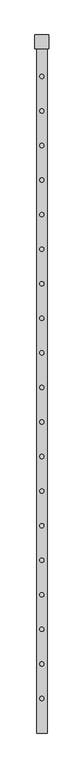
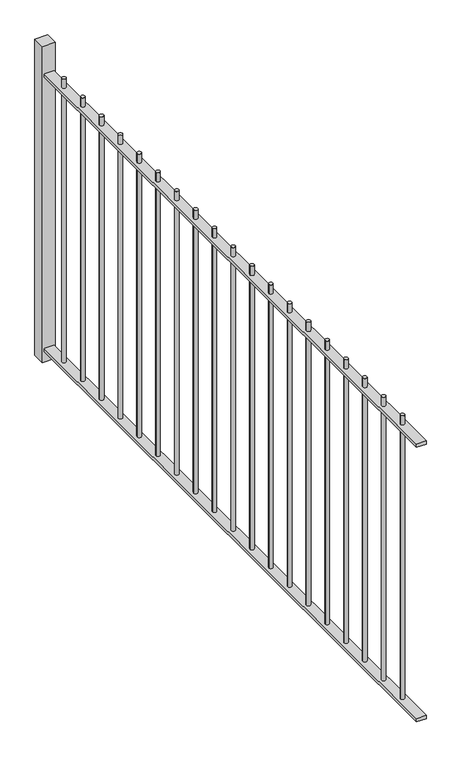
"""IFC4 building model written with IfcOpenShell, lengths in millimetres: railing geometry."""

from ifc_helpers import new_model, si_unit, point, frame, frame_2d, origin, place, context, project, spatial, polyline, circle_curve, trimmed, segment, composite_curve, outline, extrude, source, transform, mapped, element, save


def railing_8eb08526(model_context):
    return source(origin(), model_context, "Body", "SweptSolid", [
        extrude(outline(polyline([(-6549.419961, -16851.1119119), (-6489.419961, -16851.1119119), (-6489.419961, -20851.1119119), (-6549.419961, -20851.1119119), (-6549.419961, -16851.1119119)])), frame((0.0, 0.0, -30.0), z_axis=(0.0, 0.0, 1.0), x_axis=(1.0, 0.0, 0.0)), (0.0, 0.0, 1.0), 20.0),
        extrude(outline(polyline([(-6549.419961, -16851.1119119), (-6489.419961, -16851.1119119), (-6489.419961, -20851.1119119), (-6549.419961, -20851.1119119), (-6549.419961, -16851.1119119)])), frame((0.0, 0.0, 1750.0), z_axis=(0.0, 0.0, 1.0), x_axis=(1.0, 0.0, 0.0)), (0.0, 0.0, 1.0), 20.0),
        extrude(outline(composite_curve([segment(trimmed(circle_curve(frame_2d((-6519.419961, -20651.1119119)), 12.5), [point((-6531.919961, -20651.1119119))], [point((-6506.919961, -20651.1119119))], False, "CARTESIAN"), True, "CONTINUOUS"), segment(trimmed(circle_curve(frame_2d((-6519.419961, -20651.1119119)), 12.5), [point((-6506.919961, -20651.1119119))], [point((-6531.919961, -20651.1119119))], False, "CARTESIAN"), True, "CONTINUOUS")], self_intersect=False)), frame((0.0, 0.0, -10.0), z_axis=(0.0, 0.0, 1.0), x_axis=(1.0, 0.0, 0.0)), (0.0, 0.0, 1.0), 1840.0),
        extrude(outline(composite_curve([segment(trimmed(circle_curve(frame_2d((-6519.419961, -20451.1119119)), 12.5), [point((-6531.919961, -20451.1119119))], [point((-6506.919961, -20451.1119119))], False, "CARTESIAN"), True, "CONTINUOUS"), segment(trimmed(circle_curve(frame_2d((-6519.419961, -20451.1119119)), 12.5), [point((-6506.919961, -20451.1119119))], [point((-6531.919961, -20451.1119119))], False, "CARTESIAN"), True, "CONTINUOUS")], self_intersect=False)), frame((0.0, 0.0, -10.0), z_axis=(0.0, 0.0, 1.0), x_axis=(1.0, 0.0, 0.0)), (0.0, 0.0, 1.0), 1840.0),
        extrude(outline(composite_curve([segment(trimmed(circle_curve(frame_2d((-6519.419961, -20251.1119119)), 12.5), [point((-6531.919961, -20251.1119119))], [point((-6506.919961, -20251.1119119))], False, "CARTESIAN"), True, "CONTINUOUS"), segment(trimmed(circle_curve(frame_2d((-6519.419961, -20251.1119119)), 12.5), [point((-6506.919961, -20251.1119119))], [point((-6531.919961, -20251.1119119))], False, "CARTESIAN"), True, "CONTINUOUS")], self_intersect=False)), frame((0.0, 0.0, -10.0), z_axis=(0.0, 0.0, 1.0), x_axis=(1.0, 0.0, 0.0)), (0.0, 0.0, 1.0), 1840.0),
        extrude(outline(composite_curve([segment(trimmed(circle_curve(frame_2d((-6519.419961, -20051.1119119)), 12.5), [point((-6531.919961, -20051.1119119))], [point((-6506.919961, -20051.1119119))], False, "CARTESIAN"), True, "CONTINUOUS"), segment(trimmed(circle_curve(frame_2d((-6519.419961, -20051.1119119)), 12.5), [point((-6506.919961, -20051.1119119))], [point((-6531.919961, -20051.1119119))], False, "CARTESIAN"), True, "CONTINUOUS")], self_intersect=False)), frame((0.0, 0.0, -10.0), z_axis=(0.0, 0.0, 1.0), x_axis=(1.0, 0.0, 0.0)), (0.0, 0.0, 1.0), 1840.0),
        extrude(outline(composite_curve([segment(trimmed(circle_curve(frame_2d((-6519.419961, -19851.1119119)), 12.5), [point((-6531.919961, -19851.1119119))], [point((-6506.919961, -19851.1119119))], False, "CARTESIAN"), True, "CONTINUOUS"), segment(trimmed(circle_curve(frame_2d((-6519.419961, -19851.1119119)), 12.5), [point((-6506.919961, -19851.1119119))], [point((-6531.919961, -19851.1119119))], False, "CARTESIAN"), True, "CONTINUOUS")], self_intersect=False)), frame((0.0, 0.0, -10.0), z_axis=(0.0, 0.0, 1.0), x_axis=(1.0, 0.0, 0.0)), (0.0, 0.0, 1.0), 1840.0),
        extrude(outline(composite_curve([segment(trimmed(circle_curve(frame_2d((-6519.419961, -19651.1119119)), 12.5), [point((-6531.919961, -19651.1119119))], [point((-6506.919961, -19651.1119119))], False, "CARTESIAN"), True, "CONTINUOUS"), segment(trimmed(circle_curve(frame_2d((-6519.419961, -19651.1119119)), 12.5), [point((-6506.919961, -19651.1119119))], [point((-6531.919961, -19651.1119119))], False, "CARTESIAN"), True, "CONTINUOUS")], self_intersect=False)), frame((0.0, 0.0, -10.0), z_axis=(0.0, 0.0, 1.0), x_axis=(1.0, 0.0, 0.0)), (0.0, 0.0, 1.0), 1840.0),
        extrude(outline(composite_curve([segment(trimmed(circle_curve(frame_2d((-6519.419961, -19451.1119119)), 12.5), [point((-6531.919961, -19451.1119119))], [point((-6506.919961, -19451.1119119))], False, "CARTESIAN"), True, "CONTINUOUS"), segment(trimmed(circle_curve(frame_2d((-6519.419961, -19451.1119119)), 12.5), [point((-6506.919961, -19451.1119119))], [point((-6531.919961, -19451.1119119))], False, "CARTESIAN"), True, "CONTINUOUS")], self_intersect=False)), frame((0.0, 0.0, -10.0), z_axis=(0.0, 0.0, 1.0), x_axis=(1.0, 0.0, 0.0)), (0.0, 0.0, 1.0), 1840.0),
        extrude(outline(composite_curve([segment(trimmed(circle_curve(frame_2d((-6519.419961, -19251.1119119)), 12.5), [point((-6531.919961, -19251.1119119))], [point((-6506.919961, -19251.1119119))], False, "CARTESIAN"), True, "CONTINUOUS"), segment(trimmed(circle_curve(frame_2d((-6519.419961, -19251.1119119)), 12.5), [point((-6506.919961, -19251.1119119))], [point((-6531.919961, -19251.1119119))], False, "CARTESIAN"), True, "CONTINUOUS")], self_intersect=False)), frame((0.0, 0.0, -10.0), z_axis=(0.0, 0.0, 1.0), x_axis=(1.0, 0.0, 0.0)), (0.0, 0.0, 1.0), 1840.0),
        extrude(outline(composite_curve([segment(trimmed(circle_curve(frame_2d((-6519.419961, -19051.1119119)), 12.5), [point((-6531.919961, -19051.1119119))], [point((-6506.919961, -19051.1119119))], False, "CARTESIAN"), True, "CONTINUOUS"), segment(trimmed(circle_curve(frame_2d((-6519.419961, -19051.1119119)), 12.5), [point((-6506.919961, -19051.1119119))], [point((-6531.919961, -19051.1119119))], False, "CARTESIAN"), True, "CONTINUOUS")], self_intersect=False)), frame((0.0, 0.0, -10.0), z_axis=(0.0, 0.0, 1.0), x_axis=(1.0, 0.0, 0.0)), (0.0, 0.0, 1.0), 1840.0),
        extrude(outline(composite_curve([segment(trimmed(circle_curve(frame_2d((-6519.419961, -18851.1119119)), 12.5), [point((-6531.919961, -18851.1119119))], [point((-6506.919961, -18851.1119119))], False, "CARTESIAN"), True, "CONTINUOUS"), segment(trimmed(circle_curve(frame_2d((-6519.419961, -18851.1119119)), 12.5), [point((-6506.919961, -18851.1119119))], [point((-6531.919961, -18851.1119119))], False, "CARTESIAN"), True, "CONTINUOUS")], self_intersect=False)), frame((0.0, 0.0, -10.0), z_axis=(0.0, 0.0, 1.0), x_axis=(1.0, 0.0, 0.0)), (0.0, 0.0, 1.0), 1840.0),
        extrude(outline(composite_curve([segment(trimmed(circle_curve(frame_2d((-6519.419961, -18651.1119119)), 12.5), [point((-6531.919961, -18651.1119119))], [point((-6506.919961, -18651.1119119))], False, "CARTESIAN"), True, "CONTINUOUS"), segment(trimmed(circle_curve(frame_2d((-6519.419961, -18651.1119119)), 12.5), [point((-6506.919961, -18651.1119119))], [point((-6531.919961, -18651.1119119))], False, "CARTESIAN"), True, "CONTINUOUS")], self_intersect=False)), frame((0.0, 0.0, -10.0), z_axis=(0.0, 0.0, 1.0), x_axis=(1.0, 0.0, 0.0)), (0.0, 0.0, 1.0), 1840.0),
        extrude(outline(composite_curve([segment(trimmed(circle_curve(frame_2d((-6519.419961, -18451.1119119)), 12.5), [point((-6531.919961, -18451.1119119))], [point((-6506.919961, -18451.1119119))], False, "CARTESIAN"), True, "CONTINUOUS"), segment(trimmed(circle_curve(frame_2d((-6519.419961, -18451.1119119)), 12.5), [point((-6506.919961, -18451.1119119))], [point((-6531.919961, -18451.1119119))], False, "CARTESIAN"), True, "CONTINUOUS")], self_intersect=False)), frame((0.0, 0.0, -10.0), z_axis=(0.0, 0.0, 1.0), x_axis=(1.0, 0.0, 0.0)), (0.0, 0.0, 1.0), 1840.0),
        extrude(outline(composite_curve([segment(trimmed(circle_curve(frame_2d((-6519.419961, -18251.1119119)), 12.5), [point((-6531.919961, -18251.1119119))], [point((-6506.919961, -18251.1119119))], False, "CARTESIAN"), True, "CONTINUOUS"), segment(trimmed(circle_curve(frame_2d((-6519.419961, -18251.1119119)), 12.5), [point((-6506.919961, -18251.1119119))], [point((-6531.919961, -18251.1119119))], False, "CARTESIAN"), True, "CONTINUOUS")], self_intersect=False)), frame((0.0, 0.0, -10.0), z_axis=(0.0, 0.0, 1.0), x_axis=(1.0, 0.0, 0.0)), (0.0, 0.0, 1.0), 1840.0),
        extrude(outline(composite_curve([segment(trimmed(circle_curve(frame_2d((-6519.419961, -18051.1119119)), 12.5), [point((-6531.919961, -18051.1119119))], [point((-6506.919961, -18051.1119119))], False, "CARTESIAN"), True, "CONTINUOUS"), segment(trimmed(circle_curve(frame_2d((-6519.419961, -18051.1119119)), 12.5), [point((-6506.919961, -18051.1119119))], [point((-6531.919961, -18051.1119119))], False, "CARTESIAN"), True, "CONTINUOUS")], self_intersect=False)), frame((0.0, 0.0, -10.0), z_axis=(0.0, 0.0, 1.0), x_axis=(1.0, 0.0, 0.0)), (0.0, 0.0, 1.0), 1840.0),
        extrude(outline(composite_curve([segment(trimmed(circle_curve(frame_2d((-6519.419961, -17851.1119119)), 12.5), [point((-6531.919961, -17851.1119119))], [point((-6506.919961, -17851.1119119))], False, "CARTESIAN"), True, "CONTINUOUS"), segment(trimmed(circle_curve(frame_2d((-6519.419961, -17851.1119119)), 12.5), [point((-6506.919961, -17851.1119119))], [point((-6531.919961, -17851.1119119))], False, "CARTESIAN"), True, "CONTINUOUS")], self_intersect=False)), frame((0.0, 0.0, -10.0), z_axis=(0.0, 0.0, 1.0), x_axis=(1.0, 0.0, 0.0)), (0.0, 0.0, 1.0), 1840.0),
        extrude(outline(composite_curve([segment(trimmed(circle_curve(frame_2d((-6519.419961, -17651.1119119)), 12.5), [point((-6531.919961, -17651.1119119))], [point((-6506.919961, -17651.1119119))], False, "CARTESIAN"), True, "CONTINUOUS"), segment(trimmed(circle_curve(frame_2d((-6519.419961, -17651.1119119)), 12.5), [point((-6506.919961, -17651.1119119))], [point((-6531.919961, -17651.1119119))], False, "CARTESIAN"), True, "CONTINUOUS")], self_intersect=False)), frame((0.0, 0.0, -10.0), z_axis=(0.0, 0.0, 1.0), x_axis=(1.0, 0.0, 0.0)), (0.0, 0.0, 1.0), 1840.0),
        extrude(outline(composite_curve([segment(trimmed(circle_curve(frame_2d((-6519.419961, -17451.1119119)), 12.5), [point((-6531.919961, -17451.1119119))], [point((-6506.919961, -17451.1119119))], False, "CARTESIAN"), True, "CONTINUOUS"), segment(trimmed(circle_curve(frame_2d((-6519.419961, -17451.1119119)), 12.5), [point((-6506.919961, -17451.1119119))], [point((-6531.919961, -17451.1119119))], False, "CARTESIAN"), True, "CONTINUOUS")], self_intersect=False)), frame((0.0, 0.0, -10.0), z_axis=(0.0, 0.0, 1.0), x_axis=(1.0, 0.0, 0.0)), (0.0, 0.0, 1.0), 1840.0),
        extrude(outline(composite_curve([segment(trimmed(circle_curve(frame_2d((-6519.419961, -17251.1119119)), 12.5), [point((-6531.919961, -17251.1119119))], [point((-6506.919961, -17251.1119119))], False, "CARTESIAN"), True, "CONTINUOUS"), segment(trimmed(circle_curve(frame_2d((-6519.419961, -17251.1119119)), 12.5), [point((-6506.919961, -17251.1119119))], [point((-6531.919961, -17251.1119119))], False, "CARTESIAN"), True, "CONTINUOUS")], self_intersect=False)), frame((0.0, 0.0, -10.0), z_axis=(0.0, 0.0, 1.0), x_axis=(1.0, 0.0, 0.0)), (0.0, 0.0, 1.0), 1840.0),
        extrude(outline(composite_curve([segment(trimmed(circle_curve(frame_2d((-6519.419961, -17051.1119119)), 12.5), [point((-6531.919961, -17051.1119119))], [point((-6506.919961, -17051.1119119))], False, "CARTESIAN"), True, "CONTINUOUS"), segment(trimmed(circle_curve(frame_2d((-6519.419961, -17051.1119119)), 12.5), [point((-6506.919961, -17051.1119119))], [point((-6531.919961, -17051.1119119))], False, "CARTESIAN"), True, "CONTINUOUS")], self_intersect=False)), frame((0.0, 0.0, -10.0), z_axis=(0.0, 0.0, 1.0), x_axis=(1.0, 0.0, 0.0)), (0.0, 0.0, 1.0), 1840.0),
        extrude(outline(polyline([(-6479.419961, -16811.1119119), (-6479.419961, -16891.1119119), (-6559.419961, -16891.1119119), (-6559.419961, -16811.1119119), (-6479.419961, -16811.1119119)])), frame((0.0, 0.0, -100.0), z_axis=(0.0, 0.0, 1.0), x_axis=(1.0, 0.0, 0.0)), (0.0, 0.0, 1.0), 2050.0),
    ])


if __name__ == "__main__":
    model = new_model("IFC4")
    model_context = context("Model", 3, world=origin())
    ifc_project = project(units=[si_unit("LENGTHUNIT", "METRE", prefix="MILLI")], contexts=[model_context])
    site = spatial("IfcSite", under=ifc_project)
    building = spatial("IfcBuilding", under=site)
    placement = place(None, origin())
    railing_shape = railing_8eb08526(model_context)
    element("IfcRailing", 1, at=placement, inside=building, context=model_context, shape_type="MappedRepresentation", body=[
        mapped(railing_shape, transform((0.0, 0.0, 0.0), x_axis=(1.0, 0.0, 0.0), y_axis=(0.0, 1.0, 0.0), z_axis=(0.0, 0.0, 1.0))),
    ])
    save(model, "model.ifc")

# Revit data of these elements
# Element 1 (IfcRailing)
#   Materials on its faces: "NLRS_h2_staal_generiek zwart_gen_rsf", "NLRS_h2_staal_gen_rsf"
# Materials
#   "NLRS_h2_staal_generiek zwart_gen_rsf": class "Metal", colour RGB 189 187 185, transparency 0, Manufacturer = "RevitGG", URL = "www.revitgg.nl", Description = "Staal, generiek materiaal", Cost = 0
#   "NLRS_h2_staal_gen_rsf": class "H - Metaal", colour RGB 189 187 185, transparency 0, Keynote = "h2", Model = "generiek", Manufacturer = "Revit Standards Foundation", URL = "www.revitstandards.org", Description = "staal", Cost = 0
